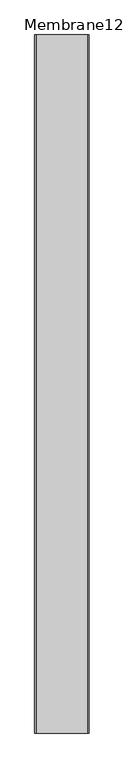
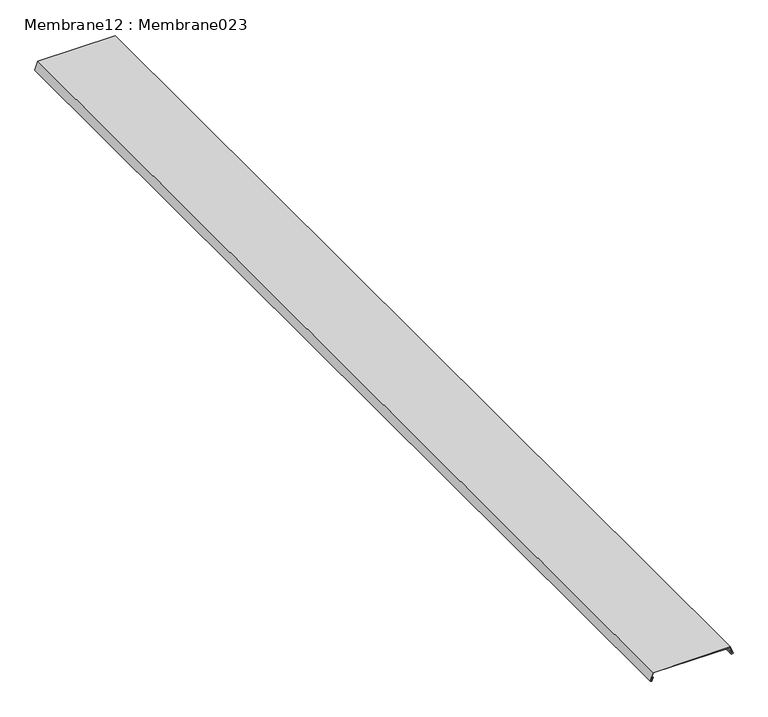
"""IFC4 building model written with IfcOpenShell, lengths in millimetres: proxy geometry, Membrane12 : Membrane023."""

from ifc_helpers import new_model, si_unit, frame, origin, place, context, project, spatial, polyline, outline, extrude, source, transform, mapped, element, save


def membrane12_membrane023_de37822b(model_context):
    return source(origin(), model_context, "Body", "SweptSolid", [
        extrude(outline(polyline([(40125.2594856, -9922.1042501), (40109.8939799, -9927.6968368), (40108.6896714, -9924.3880263), (40115.8585035, -9921.7787849), (40116.2005236, -9922.7184775), (40109.9713842, -9924.9856988), (40110.4916524, -9926.415124), (40124.2594856, -9921.4040425), (40124.2594856, -9777.6091521), (40112.0732189, -9773.1737137), (40111.5529506, -9774.6031389), (40117.7820901, -9776.8703603), (40117.4400699, -9777.8100529), (40110.2712379, -9775.2008114), (40111.4755464, -9771.892001), (40125.2594856, -9776.9089446), (40125.2594856, -9922.1042501)])), frame((0.0, 7182.1531721, 0.0), z_axis=(0.0, 1.0, 0.0), x_axis=(0.0, 0.0, 1.0)), (0.0, 0.0, 1.0), 2000.0),
    ])


if __name__ == "__main__":
    model = new_model("IFC4")
    model_context = context("Model", 3, world=origin())
    ifc_project = project(units=[si_unit("LENGTHUNIT", "METRE", prefix="MILLI")], contexts=[model_context])
    site = spatial("IfcSite", under=ifc_project)
    building = spatial("IfcBuilding", under=site)
    placement = place(None, origin())
    membrane12_membrane023_shape = membrane12_membrane023_de37822b(model_context)
    element("IfcBuildingElementProxy", 1, Name="Membrane12 : Membrane023", ObjectType="Membrane12 : Membrane023", at=placement, inside=building, context=model_context, shape_type="MappedRepresentation", body=[
        mapped(membrane12_membrane023_shape, transform((0.0, 0.0, 0.0), x_axis=(1.0, 0.0, 0.0), y_axis=(0.0, 1.0, 0.0), z_axis=(0.0, 0.0, 1.0))),
    ])
    save(model, "model.ifc")

# Revit data of these elements
# Type "Membrane12 : Membrane023"
#   NameOverride = "Membrane023"
# Element 1 (IfcBuildingElementProxy, "Membrane12 : Membrane023")
#   Materials on its faces: "16 GA. COPPER FLASHING"
# Materials
#   "16 GA. COPPER FLASHING": class "Unassigned", colour RGB 251 232 155, transparency 0, Cost = 0
